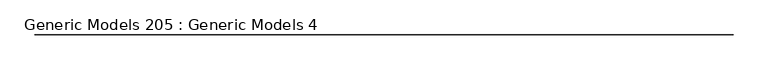
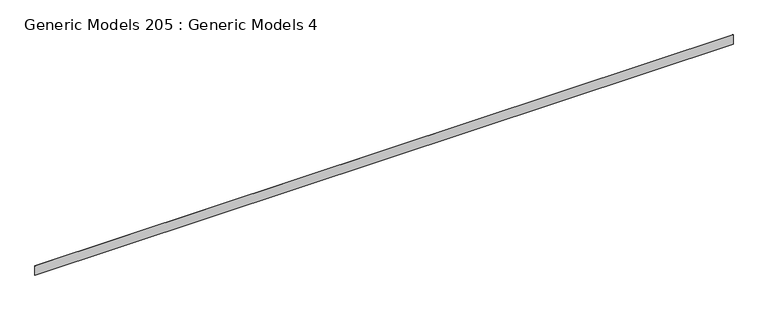
"""IFC4 building model written with IfcOpenShell, lengths in millimetres: proxy geometry, Generic Models 205 : Generic Models 4."""

from ifc_helpers import new_model, si_unit, frame, origin, place, context, project, spatial, polyline, outline, extrude, source, transform, mapped, element, save


def generic_models_205_generic_models_4_30cdf4a9(model_context):
    return source(origin(), model_context, "Body", "SweptSolid", [
        extrude(outline(polyline([(2196.9263704, -5467.9765747), (2196.9263704, -5468.7703247), (-10234.5171316, -5468.7703247), (-10234.5171316, -5467.9765747), (2196.9263704, -5467.9765747)])), frame((0.0, 0.0, 126181.6443718), z_axis=(0.0, 0.0, 1.0), x_axis=(1.0, 0.0, 0.0)), (0.0, 0.0, 1.0), 177.4438364),
    ])


if __name__ == "__main__":
    model = new_model("IFC4")
    model_context = context("Model", 3, world=origin())
    ifc_project = project(units=[si_unit("LENGTHUNIT", "METRE", prefix="MILLI")], contexts=[model_context])
    site = spatial("IfcSite", under=ifc_project)
    building = spatial("IfcBuilding", under=site)
    placement = place(None, origin())
    generic_models_205_generic_models_4_shape = generic_models_205_generic_models_4_30cdf4a9(model_context)
    element("IfcBuildingElementProxy", 1, Name="Generic Models 205 : Generic Models 4", ObjectType="Generic Models 205 : Generic Models 4", at=placement, inside=building, context=model_context, shape_type="MappedRepresentation", body=[
        mapped(generic_models_205_generic_models_4_shape, transform((0.0, 0.0, 0.0), x_axis=(1.0, 0.0, 0.0), y_axis=(0.0, 1.0, 0.0), z_axis=(0.0, 0.0, 1.0))),
    ])
    save(model, "model.ifc")

# Revit data of these elements
# Element 1 (IfcBuildingElementProxy, "Generic Models 205 : Generic Models 4")
#   Materials on its faces: "_(2) LAYERS NO. 30 ASTM D226 ASPHALT SATURATED ORGANIC FELT"
# Materials
#   "_(2) LAYERS NO. 30 ASTM D226 ASPHALT SATURATED ORGANIC FELT": class "Generic", colour RGB 67 154 161, transparency 0, Cost = 0
